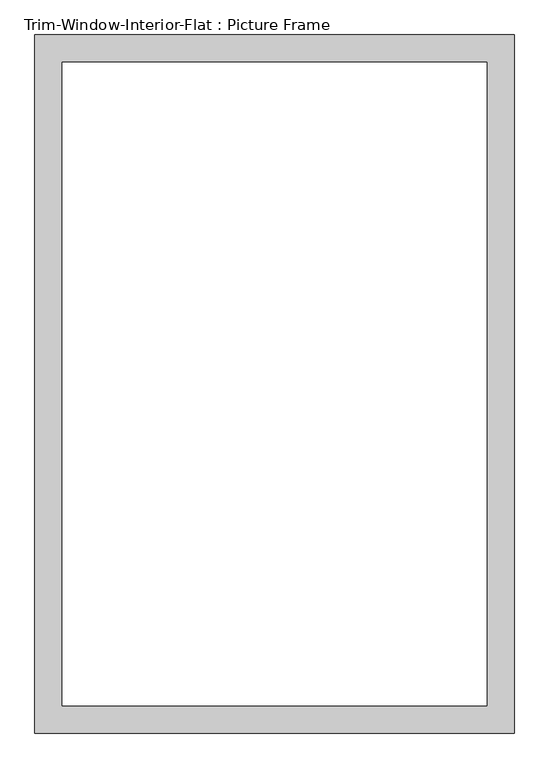
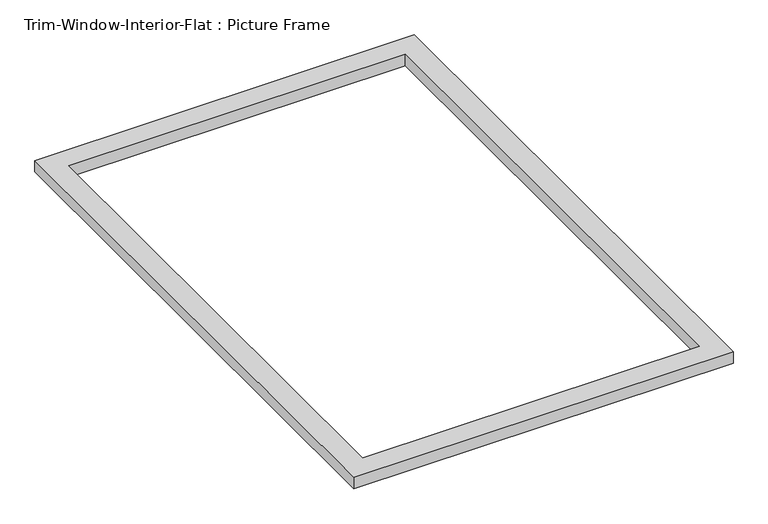
"""IFC4 building model written with IfcOpenShell, lengths in millimetres: proxy geometry, Trim-Window-Interior-Flat : Picture Frame."""

import ifcopenshell
import ifcopenshell.guid

model = None  # the IFC model being written
_history = None  # IfcOwnerHistory: only IFC2X3 demands one
_inside = {}  # id of a spatial element -> (the spatial element, [elements in it])
_under = {}  # id of a project, library or spatial element -> (it, [spatial elements below it])
_declared = {}  # id of a project -> (the project, [libraries it declares])
_typed = {}  # id of a type object -> (the type object, [elements of that type])
_made_of = {}  # id of a material, layer set ... -> (it, [elements and type objects made of it])


def new_model(schema):
    """Start an empty IFC model of exactly this schema.

    Asked for "IFC4X3", IfcOpenShell would pick the latest addendum, in which some entities
    have other attributes; the version numbers below select the first issue.
    IFC2X3 requires an IfcOwnerHistory on every rooted entity: one is made here for all.
    """
    global model, _history
    if schema == "IFC4X3":
        model = ifcopenshell.file(schema_version=(4, 3, 0, 0))
    else:
        model = ifcopenshell.file(schema=schema)
    _inside.clear()
    _under.clear()
    _declared.clear()
    _typed.clear()
    _made_of.clear()
    _history = None
    if model.schema == "IFC2X3":
        org = make("IfcOrganization", Name="unknown")
        user = make(
            "IfcPersonAndOrganization",
            ThePerson=make("IfcPerson", FamilyName="unknown"),
            TheOrganization=org,
        )
        app = make(
            "IfcApplication",
            ApplicationDeveloper=org,
            Version="unknown",
            ApplicationFullName="unknown",
            ApplicationIdentifier="unknown",
        )
        _history = make(
            "IfcOwnerHistory",
            OwningUser=user,
            OwningApplication=app,
            ChangeAction="ADDED",
            CreationDate=0,
        )
    return model


def make(cls, **values):
    """One entity of the class cls with the attributes given. An attribute that is None is left unset."""
    return model.create_entity(
        cls, **{name: value for name, value in values.items() if value is not None}
    )


def rooted(cls, **values):
    """An entity with a GlobalId (a new one), such as an element, a storey or a relation."""
    return make(cls, GlobalId=ifcopenshell.guid.new(), OwnerHistory=_history, **values)


def si_unit(unit_type, name, prefix=None):
    """IfcSIUnit, for example si_unit("LENGTHUNIT", "METRE", prefix="MILLI")."""
    return make("IfcSIUnit", UnitType=unit_type, Prefix=prefix, Name=name)


def assignment(units):
    """IfcUnitAssignment: the units of a project."""
    return None if units is None else make("IfcUnitAssignment", Units=units)


def point(xyz):
    """IfcCartesianPoint."""
    return None if xyz is None else make("IfcCartesianPoint", Coordinates=xyz)


def direction(xyz):
    """IfcDirection."""
    return None if xyz is None else make("IfcDirection", DirectionRatios=xyz)


def frame(location, z_axis=None, x_axis=None):
    """IfcAxis2Placement3D, a coordinate frame: its origin and axes. An axis left out is left unset."""
    return make(
        "IfcAxis2Placement3D",
        Location=point(location),
        Axis=direction(z_axis),
        RefDirection=direction(x_axis),
    )


def origin():
    """The frame at (0, 0, 0) with its axes left unset."""
    return frame((0.0, 0.0, 0.0))


def origin_with_axes():
    """The frame at (0, 0, 0) with the z axis (0, 0, 1) and the x axis (1, 0, 0) written out."""
    return frame((0.0, 0.0, 0.0), z_axis=(0.0, 0.0, 1.0), x_axis=(1.0, 0.0, 0.0))


def place(relative_to, where):
    """IfcLocalPlacement: puts the frame where relative to a parent placement (None: the world)."""
    return make(
        "IfcLocalPlacement", PlacementRelTo=relative_to, RelativePlacement=where
    )


def context(
    kind, dimensions, precision=None, world=None, true_north=None, identifier=None
):
    """IfcGeometricRepresentationContext, for example the 3D "Model" context."""
    return make(
        "IfcGeometricRepresentationContext",
        ContextIdentifier=identifier,
        ContextType=kind,
        CoordinateSpaceDimension=dimensions,
        Precision=precision,
        WorldCoordinateSystem=world,
        TrueNorth=true_north,
    )


def project(units=None, contexts=None):
    """IfcProject with its units and contexts."""
    return rooted(
        "IfcProject",
        Name="project",
        RepresentationContexts=contexts,
        UnitsInContext=assignment(units),
    )


def spatial(cls, under=None, at=None, **own):
    """A site, building, storey or space (cls), placed at a placement, below another one or the project."""
    s = rooted(cls, ObjectPlacement=at, **own)
    if under is not None:
        _under.setdefault(under.id(), (under, []))[1].append(s)
    return s


def polyline(points):
    """IfcPolyline through the points."""
    return make("IfcPolyline", Points=[point(p) for p in points])


def outline(outer, holes=None, kind="AREA"):
    """IfcArbitraryClosedProfileDef: a profile drawn as a closed curve; with holes, ...WithVoids."""
    if holes is None:
        return make("IfcArbitraryClosedProfileDef", ProfileType=kind, OuterCurve=outer)
    return make(
        "IfcArbitraryProfileDefWithVoids",
        ProfileType=kind,
        OuterCurve=outer,
        InnerCurves=holes,
    )


def extrude(swept, where, along, depth):
    """IfcExtrudedAreaSolid: the profile swept, set in the frame where, extruded along a direction by depth."""
    return make(
        "IfcExtrudedAreaSolid",
        SweptArea=swept,
        Position=where,
        ExtrudedDirection=direction(along),
        Depth=depth,
    )


def shape(context_of_items, identifier, shape_type, items):
    """IfcShapeRepresentation: the items that make up one representation, for example the "Body"."""
    return make(
        "IfcShapeRepresentation",
        ContextOfItems=context_of_items,
        RepresentationIdentifier=identifier,
        RepresentationType=shape_type,
        Items=items,
    )


def source(mapping_origin, context_of_items, identifier, shape_type, items):
    """IfcRepresentationMap: a shape defined once, which mapped items show again and again."""
    return make(
        "IfcRepresentationMap",
        MappingOrigin=mapping_origin,
        MappedRepresentation=shape(context_of_items, identifier, shape_type, items),
    )


def transform(
    local_origin,
    x_axis=None,
    y_axis=None,
    z_axis=None,
    scale=None,
    scale2=None,
    scale3=None,
    uniform=True,
):
    """IfcCartesianTransformationOperator3D, or its non-uniform kind. x_axis, y_axis, z_axis: its Axis1, 2, 3."""
    if uniform:
        return make(
            "IfcCartesianTransformationOperator3D",
            Axis1=direction(x_axis),
            Axis2=direction(y_axis),
            LocalOrigin=point(local_origin),
            Scale=scale,
            Axis3=direction(z_axis),
        )
    return make(
        "IfcCartesianTransformationOperator3DnonUniform",
        Axis1=direction(x_axis),
        Axis2=direction(y_axis),
        LocalOrigin=point(local_origin),
        Scale=scale,
        Axis3=direction(z_axis),
        Scale2=scale2,
        Scale3=scale3,
    )


def mapped(mapping_source, mapping_target):
    """IfcMappedItem: shows the shape of a source again, moved by a transform."""
    return make(
        "IfcMappedItem", MappingSource=mapping_source, MappingTarget=mapping_target
    )


def made_of(thing, what):
    """Note that an element or type object is made of a material, layer set ...; save() writes the relation."""
    if what is not None:
        _made_of.setdefault(what.id(), (what, []))[1].append(thing)
    return thing


def element(
    cls,
    number,
    at=None,
    inside=None,
    cuts=None,
    type_object=None,
    material=None,
    context=None,
    identifier="Body",
    shape_type=None,
    held_by="IfcProductDefinitionShape",
    body=None,
    shapes=None,
    **own,
):
    """One element of the class cls, such as IfcWall. Its Tag is "e" and its number.

    at: its placement. inside: the storey or other place that contains it. cuts: it is an
    opening in that element (IfcRelVoidsElement). A single representation is given by context,
    identifier, shape_type and body (its items); several are given by shapes. held_by: the class
    of the entity that holds the representations. save() writes the other relations.
    """
    e = rooted(cls, Tag="e%d" % number, ObjectPlacement=at, **own)
    if body is not None:
        shapes = [shape(context, identifier, shape_type, body)]
    if shapes is not None:
        e.Representation = make(held_by, Representations=shapes)
    if inside is not None:
        _inside.setdefault(inside.id(), (inside, []))[1].append(e)
    if cuts is not None:
        rooted(
            "IfcRelVoidsElement", RelatingBuildingElement=cuts, RelatedOpeningElement=e
        )
    if type_object is not None:
        _typed.setdefault(type_object.id(), (type_object, []))[1].append(e)
    return made_of(e, material)


def aggregate(whole, parts):
    """IfcRelAggregates: a whole, such as a stair, and the parts it consists of."""
    return rooted("IfcRelAggregates", RelatingObject=whole, RelatedObjects=parts)


def save(model, path):
    """Write the relations noted so far, then the file.

    IfcRelAggregates (storeys below a building ...), IfcRelContainedInSpatialStructure (elements
    in a storey), IfcRelDefinesByType, IfcRelAssociatesMaterial and IfcRelDeclares: one each for
    every whole, place, type object, material and project.
    """
    for whole, parts in _under.values():
        aggregate(whole, parts)
    for where, things in _inside.values():
        rooted(
            "IfcRelContainedInSpatialStructure",
            RelatedElements=things,
            RelatingStructure=where,
        )
    for kind, things in _typed.values():
        rooted("IfcRelDefinesByType", RelatedObjects=things, RelatingType=kind)
    for what, things in _made_of.values():
        rooted("IfcRelAssociatesMaterial", RelatedObjects=things, RelatingMaterial=what)
    for by, libraries in _declared.values():
        rooted("IfcRelDeclares", RelatingContext=by, RelatedDefinitions=libraries)
    model.write(path)


def trim_window_interior_flat_picture_frame_edb5e600(model_context):
    return source(origin(), model_context, "Body", "SweptSolid", [
        extrude(outline(polyline([(501.65, 44.45), (501.65, -1416.05), (-501.65, -1416.05), (-501.65, 44.45), (501.65, 44.45)]), holes=[polyline([(444.5, -12.7), (-444.5, -12.7), (-444.5, -1358.9), (444.5, -1358.9), (444.5, -12.7)])]), origin_with_axes(), (0.0, 0.0, 1.0), 31.75),
    ])


if __name__ == "__main__":
    model = new_model("IFC4")
    model_context = context("Model", 3, world=origin())
    ifc_project = project(units=[si_unit("LENGTHUNIT", "METRE", prefix="MILLI")], contexts=[model_context])
    site = spatial("IfcSite", under=ifc_project)
    building = spatial("IfcBuilding", under=site)
    placement = place(None, origin())
    trim_window_interior_flat_picture_frame_shape = trim_window_interior_flat_picture_frame_edb5e600(model_context)
    element("IfcBuildingElementProxy", 1, Name="Trim-Window-Interior-Flat : Picture Frame", ObjectType="Trim-Window-Interior-Flat : Picture Frame", at=placement, inside=building, context=model_context, shape_type="MappedRepresentation", body=[
        mapped(trim_window_interior_flat_picture_frame_shape, transform((0.0, 0.0, 0.0), x_axis=(1.0, 0.0, 0.0), y_axis=(0.0, 1.0, 0.0), z_axis=(0.0, 0.0, 1.0))),
    ])
    save(model, "model.ifc")

# Revit data of these elements
# Type "Trim-Window-Interior-Flat : Picture Frame"
#   Trim Thickness_Picture Frame = 0' - 1 1/4"
#   Trim Width = 0' - 2 1/4"
#   Trim Thickness_with Sill = 0' - 0 3/4"
#   Sill Thickness = 0' - 1 1/4"
#   Opening Width [instance default] = 2' - 0"
#   Opening Height [instance default] = 3' - 0"
#   Default Elevation = 4' - 0"
#   Sill = no
#   Picture Frame = yes
#   Trim Material [instance default] = none
# Element 1 (IfcBuildingElementProxy, "Trim-Window-Interior-Flat : Picture Frame")
#   Opening Width = 3' - 0"
#   Opening Height = 4' - 6"
#   Trim Material = Wood - Stained
#   Materials on its faces: "Wood - Stained"
# Materials
#   "Wood - Stained": class "Wood", colour RGB 224 178 126, transparency 0, Cost = 0
